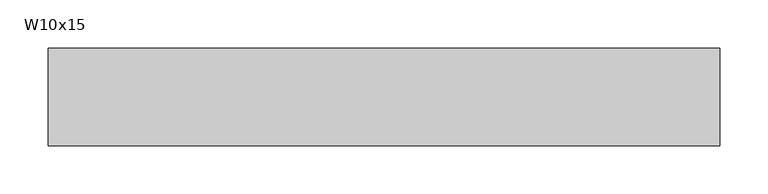
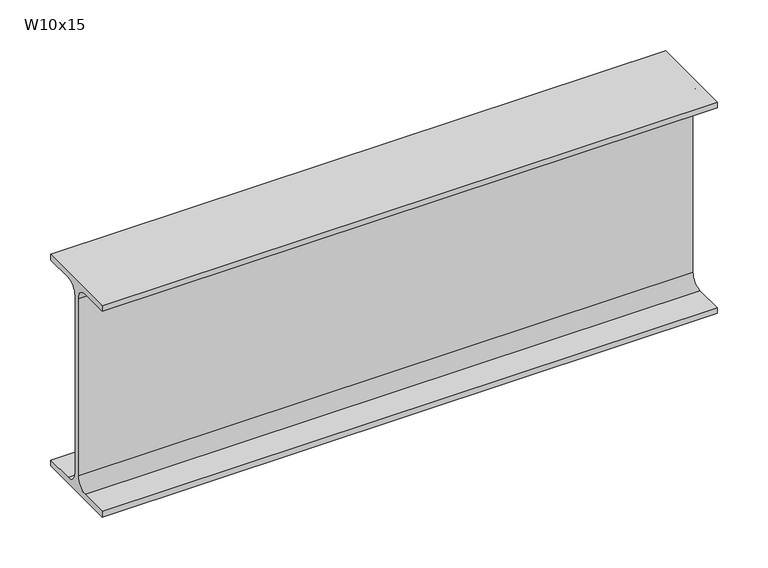
"""IFC4 building model written with IfcOpenShell, lengths in millimetres: beam geometry, RME W-Wide Flange : W10x15."""

from ifc_helpers import new_model, si_unit, point, frame, frame_2d, origin, place, context, project, spatial, polyline, circle_curve, trimmed, segment, composite_curve, outline, extrude, source, transform, mapped, element, save


def w10x15_30a09460(model_context):
    return source(origin(), model_context, "Body", "SweptSolid", [
        extrude(outline(composite_curve([segment(polyline([(50.8, -120.142), (50.8, -127.0), (-50.8, -127.0), (-50.8, -120.142), (-16.7005, -120.142)]), True, "CONTINUOUS"), segment(trimmed(circle_curve(frame_2d((-16.7005, -106.3625)), 13.7795), [point((-16.7005, -120.142))], [point((-2.921, -106.3625))], True, "CARTESIAN"), True, "CONTINUOUS"), segment(polyline([(-2.921, -106.3625), (-2.921, 106.3625)]), True, "CONTINUOUS"), segment(trimmed(circle_curve(frame_2d((-16.7005, 106.3625)), 13.7795), [point((-2.921, 106.3625))], [point((-16.7005, 120.142))], True, "CARTESIAN"), True, "CONTINUOUS"), segment(polyline([(-16.7005, 120.142), (-50.8, 120.142), (-50.8, 127.0), (50.8, 127.0), (50.8, 120.142), (16.7005, 120.142)]), True, "CONTINUOUS"), segment(trimmed(circle_curve(frame_2d((16.7005, 106.3625)), 13.7795), [point((16.7005, 120.142))], [point((2.921, 106.3625))], True, "CARTESIAN"), True, "CONTINUOUS"), segment(polyline([(2.921, 106.3625), (2.921, -106.3625)]), True, "CONTINUOUS"), segment(trimmed(circle_curve(frame_2d((16.7005, -106.3625)), 13.7795), [point((2.921, -106.3625))], [point((16.7005, -120.142))], True, "CARTESIAN"), True, "CONTINUOUS"), segment(polyline([(16.7005, -120.142), (50.8, -120.142)]), True, "CONTINUOUS")], self_intersect=False)), frame((-393.8487918, 0.0, 0.0), z_axis=(1.0, 0.0, 0.0), x_axis=(0.0, 1.0, 0.0)), (0.0, 0.0, 1.0), 698.7975836),
    ])


if __name__ == "__main__":
    model = new_model("IFC4")
    model_context = context("Model", 3, world=origin())
    ifc_project = project(units=[si_unit("LENGTHUNIT", "METRE", prefix="MILLI")], contexts=[model_context])
    site = spatial("IfcSite", under=ifc_project)
    building = spatial("IfcBuilding", under=site)
    placement = place(None, origin())
    w10x15_shape = w10x15_30a09460(model_context)
    element("IfcBeam", 1, ObjectType="RME W-Wide Flange : W10x15", at=placement, inside=building, context=model_context, shape_type="MappedRepresentation", body=[
        mapped(w10x15_shape, transform((0.0, 0.0, 0.0), x_axis=(1.0, 0.0, 0.0), y_axis=(0.0, 1.0, 0.0), z_axis=(0.0, 0.0, 1.0))),
    ])
    save(model, "model.ifc")

# Revit data of these elements
# Type "RME W-Wide Flange : W10x15"
#   WELD P [instance default] = ""
#   WELD LE [instance default] = ""
#   WELD D [instance default] = ""
#   TOP SECTION SIZE [instance default] = ""
#   TOP SECTION LENGTH [instance default] = ""
#   REMARKS [instance default] = ""
#   REINF TYPE [instance default] = ""
#   Nominal Size = "W24"
#   End Bearing Capacity [instance default] = ""
#   BOT SECTION SIZE [instance default] = ""
#   BOT SECTION LENGTH [instance default] = ""
#   Assembly Code = "B10"
#   W = 15
#   Start Extension Calculation [instance default] = 10' - 0"
#   Start Extension [instance default] = -0' - 0 1/2"
#   End Extension Calculation [instance default] = 10' - 0"
#   End Extension [instance default] = -0' - 0 1/2"
#   Length [instance default] = 5' - 0"
#   bf = 0' - 4"
#   d = 0' - 10"
#   k = 0' - 0 13/16"
#   k2 = 0' - 0.5425"
#   tf = 0' - 0.27"
#   tw = 0' - 0.23"
#   A = 0.030625 SF
#   Structural Material [instance default] = Metal - Steel - ASTM A992
# Element 1 (IfcBeam, "RME W-Wide Flange : W10x15")
#   Start Extension Calculation = 10' - 3 1/2"
#   Start Extension = 0' - 3"
#   Length = 2' - 0 3/256"
#   Materials on its faces: "Metal - Steel - ASTM A992"
# Materials
#   "Metal - Steel - ASTM A992": class "Metal", colour RGB 255 128 0, transparency 0
